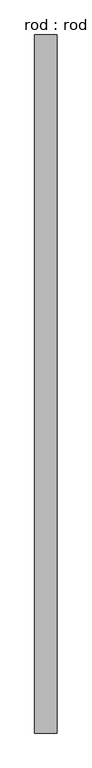
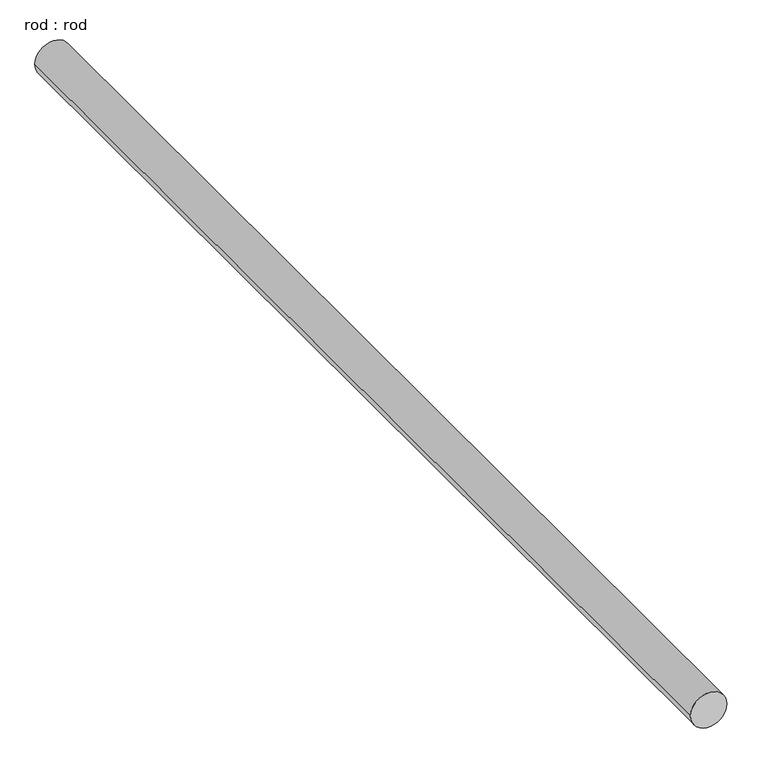
"""IFC4 building model written with IfcOpenShell, lengths in millimetres: proxy geometry, rod : rod."""

from ifc_helpers import new_model, si_unit, point, frame, frame_2d, origin, place, context, project, spatial, circle_curve, trimmed, segment, composite_curve, outline, extrude, source, transform, mapped, element, save


def rod_rod_0ea04c8a(model_context):
    return source(origin(), model_context, "Body", "SweptSolid", [
        extrude(outline(composite_curve([segment(trimmed(circle_curve(frame_2d((0.0108462, 0.0)), 200.0), [point((0.0108462, 200.0))], [point((0.0108462, -200.0))], False, "CARTESIAN"), True, "CONTINUOUS"), segment(trimmed(circle_curve(frame_2d((0.0108462, 0.0)), 200.0), [point((0.0108462, -200.0))], [point((0.0108462, 200.0))], False, "CARTESIAN"), True, "CONTINUOUS")], self_intersect=False)), frame((0.0, -2157.2713847, 0.0), z_axis=(0.0, 1.0, 0.0), x_axis=(0.0, 0.0, 1.0)), (0.0, 0.0, 1.0), 12500.0),
    ])


if __name__ == "__main__":
    model = new_model("IFC4")
    model_context = context("Model", 3, world=origin())
    ifc_project = project(units=[si_unit("LENGTHUNIT", "METRE", prefix="MILLI")], contexts=[model_context])
    site = spatial("IfcSite", under=ifc_project)
    building = spatial("IfcBuilding", under=site)
    placement = place(None, origin())
    rod_rod_shape = rod_rod_0ea04c8a(model_context)
    element("IfcBuildingElementProxy", 1, Name="rod : rod", ObjectType="rod : rod", at=placement, inside=building, context=model_context, shape_type="MappedRepresentation", body=[
        mapped(rod_rod_shape, transform((0.0, 0.0, 0.0), x_axis=(1.0, 0.0, 0.0), y_axis=(0.0, 1.0, 0.0), z_axis=(0.0, 0.0, 1.0))),
    ])
    save(model, "model.ifc")

# Revit data of these elements
# Type "rod : rod"
#   Default Elevation = 0
